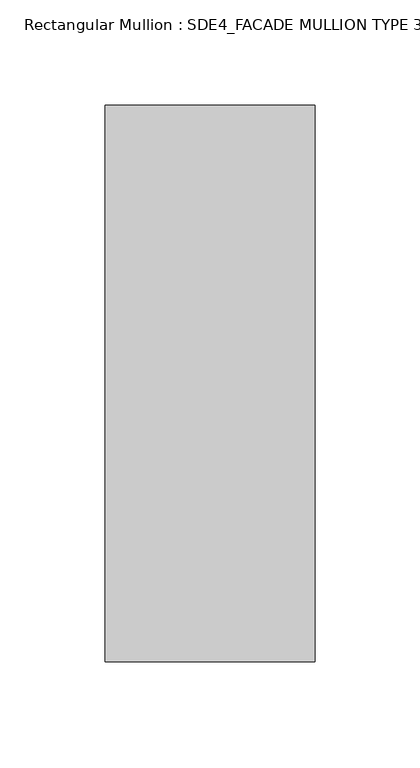
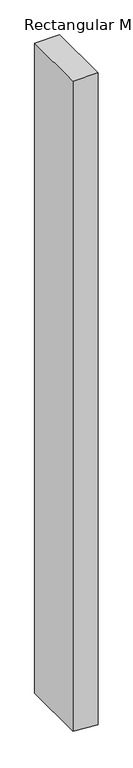
"""IFC4 building model written with IfcOpenShell, lengths in millimetres: member geometry, Rectangular Mullion : SDE4_FACADE MULLION TYPE 3."""

import ifcopenshell
import ifcopenshell.guid

model = None  # the IFC model being written
_history = None  # IfcOwnerHistory: only IFC2X3 demands one
_inside = {}  # id of a spatial element -> (the spatial element, [elements in it])
_under = {}  # id of a project, library or spatial element -> (it, [spatial elements below it])
_declared = {}  # id of a project -> (the project, [libraries it declares])
_typed = {}  # id of a type object -> (the type object, [elements of that type])
_made_of = {}  # id of a material, layer set ... -> (it, [elements and type objects made of it])


def new_model(schema):
    """Start an empty IFC model of exactly this schema.

    Asked for "IFC4X3", IfcOpenShell would pick the latest addendum, in which some entities
    have other attributes; the version numbers below select the first issue.
    IFC2X3 requires an IfcOwnerHistory on every rooted entity: one is made here for all.
    """
    global model, _history
    if schema == "IFC4X3":
        model = ifcopenshell.file(schema_version=(4, 3, 0, 0))
    else:
        model = ifcopenshell.file(schema=schema)
    _inside.clear()
    _under.clear()
    _declared.clear()
    _typed.clear()
    _made_of.clear()
    _history = None
    if model.schema == "IFC2X3":
        org = make("IfcOrganization", Name="unknown")
        user = make(
            "IfcPersonAndOrganization",
            ThePerson=make("IfcPerson", FamilyName="unknown"),
            TheOrganization=org,
        )
        app = make(
            "IfcApplication",
            ApplicationDeveloper=org,
            Version="unknown",
            ApplicationFullName="unknown",
            ApplicationIdentifier="unknown",
        )
        _history = make(
            "IfcOwnerHistory",
            OwningUser=user,
            OwningApplication=app,
            ChangeAction="ADDED",
            CreationDate=0,
        )
    return model


def make(cls, **values):
    """One entity of the class cls with the attributes given. An attribute that is None is left unset."""
    return model.create_entity(
        cls, **{name: value for name, value in values.items() if value is not None}
    )


def rooted(cls, **values):
    """An entity with a GlobalId (a new one), such as an element, a storey or a relation."""
    return make(cls, GlobalId=ifcopenshell.guid.new(), OwnerHistory=_history, **values)


def si_unit(unit_type, name, prefix=None):
    """IfcSIUnit, for example si_unit("LENGTHUNIT", "METRE", prefix="MILLI")."""
    return make("IfcSIUnit", UnitType=unit_type, Prefix=prefix, Name=name)


def assignment(units):
    """IfcUnitAssignment: the units of a project."""
    return None if units is None else make("IfcUnitAssignment", Units=units)


def point(xyz):
    """IfcCartesianPoint."""
    return None if xyz is None else make("IfcCartesianPoint", Coordinates=xyz)


def direction(xyz):
    """IfcDirection."""
    return None if xyz is None else make("IfcDirection", DirectionRatios=xyz)


def frame(location, z_axis=None, x_axis=None):
    """IfcAxis2Placement3D, a coordinate frame: its origin and axes. An axis left out is left unset."""
    return make(
        "IfcAxis2Placement3D",
        Location=point(location),
        Axis=direction(z_axis),
        RefDirection=direction(x_axis),
    )


def origin():
    """The frame at (0, 0, 0) with its axes left unset."""
    return frame((0.0, 0.0, 0.0))


def place(relative_to, where):
    """IfcLocalPlacement: puts the frame where relative to a parent placement (None: the world)."""
    return make(
        "IfcLocalPlacement", PlacementRelTo=relative_to, RelativePlacement=where
    )


def context(
    kind, dimensions, precision=None, world=None, true_north=None, identifier=None
):
    """IfcGeometricRepresentationContext, for example the 3D "Model" context."""
    return make(
        "IfcGeometricRepresentationContext",
        ContextIdentifier=identifier,
        ContextType=kind,
        CoordinateSpaceDimension=dimensions,
        Precision=precision,
        WorldCoordinateSystem=world,
        TrueNorth=true_north,
    )


def project(units=None, contexts=None):
    """IfcProject with its units and contexts."""
    return rooted(
        "IfcProject",
        Name="project",
        RepresentationContexts=contexts,
        UnitsInContext=assignment(units),
    )


def spatial(cls, under=None, at=None, **own):
    """A site, building, storey or space (cls), placed at a placement, below another one or the project."""
    s = rooted(cls, ObjectPlacement=at, **own)
    if under is not None:
        _under.setdefault(under.id(), (under, []))[1].append(s)
    return s


def polyline(points):
    """IfcPolyline through the points."""
    return make("IfcPolyline", Points=[point(p) for p in points])


def outline(outer, holes=None, kind="AREA"):
    """IfcArbitraryClosedProfileDef: a profile drawn as a closed curve; with holes, ...WithVoids."""
    if holes is None:
        return make("IfcArbitraryClosedProfileDef", ProfileType=kind, OuterCurve=outer)
    return make(
        "IfcArbitraryProfileDefWithVoids",
        ProfileType=kind,
        OuterCurve=outer,
        InnerCurves=holes,
    )


def extrude(swept, where, along, depth):
    """IfcExtrudedAreaSolid: the profile swept, set in the frame where, extruded along a direction by depth."""
    return make(
        "IfcExtrudedAreaSolid",
        SweptArea=swept,
        Position=where,
        ExtrudedDirection=direction(along),
        Depth=depth,
    )


def shape(context_of_items, identifier, shape_type, items):
    """IfcShapeRepresentation: the items that make up one representation, for example the "Body"."""
    return make(
        "IfcShapeRepresentation",
        ContextOfItems=context_of_items,
        RepresentationIdentifier=identifier,
        RepresentationType=shape_type,
        Items=items,
    )


def source(mapping_origin, context_of_items, identifier, shape_type, items):
    """IfcRepresentationMap: a shape defined once, which mapped items show again and again."""
    return make(
        "IfcRepresentationMap",
        MappingOrigin=mapping_origin,
        MappedRepresentation=shape(context_of_items, identifier, shape_type, items),
    )


def transform(
    local_origin,
    x_axis=None,
    y_axis=None,
    z_axis=None,
    scale=None,
    scale2=None,
    scale3=None,
    uniform=True,
):
    """IfcCartesianTransformationOperator3D, or its non-uniform kind. x_axis, y_axis, z_axis: its Axis1, 2, 3."""
    if uniform:
        return make(
            "IfcCartesianTransformationOperator3D",
            Axis1=direction(x_axis),
            Axis2=direction(y_axis),
            LocalOrigin=point(local_origin),
            Scale=scale,
            Axis3=direction(z_axis),
        )
    return make(
        "IfcCartesianTransformationOperator3DnonUniform",
        Axis1=direction(x_axis),
        Axis2=direction(y_axis),
        LocalOrigin=point(local_origin),
        Scale=scale,
        Axis3=direction(z_axis),
        Scale2=scale2,
        Scale3=scale3,
    )


def mapped(mapping_source, mapping_target):
    """IfcMappedItem: shows the shape of a source again, moved by a transform."""
    return make(
        "IfcMappedItem", MappingSource=mapping_source, MappingTarget=mapping_target
    )


def made_of(thing, what):
    """Note that an element or type object is made of a material, layer set ...; save() writes the relation."""
    if what is not None:
        _made_of.setdefault(what.id(), (what, []))[1].append(thing)
    return thing


def element(
    cls,
    number,
    at=None,
    inside=None,
    cuts=None,
    type_object=None,
    material=None,
    context=None,
    identifier="Body",
    shape_type=None,
    held_by="IfcProductDefinitionShape",
    body=None,
    shapes=None,
    **own,
):
    """One element of the class cls, such as IfcWall. Its Tag is "e" and its number.

    at: its placement. inside: the storey or other place that contains it. cuts: it is an
    opening in that element (IfcRelVoidsElement). A single representation is given by context,
    identifier, shape_type and body (its items); several are given by shapes. held_by: the class
    of the entity that holds the representations. save() writes the other relations.
    """
    e = rooted(cls, Tag="e%d" % number, ObjectPlacement=at, **own)
    if body is not None:
        shapes = [shape(context, identifier, shape_type, body)]
    if shapes is not None:
        e.Representation = make(held_by, Representations=shapes)
    if inside is not None:
        _inside.setdefault(inside.id(), (inside, []))[1].append(e)
    if cuts is not None:
        rooted(
            "IfcRelVoidsElement", RelatingBuildingElement=cuts, RelatedOpeningElement=e
        )
    if type_object is not None:
        _typed.setdefault(type_object.id(), (type_object, []))[1].append(e)
    return made_of(e, material)


def aggregate(whole, parts):
    """IfcRelAggregates: a whole, such as a stair, and the parts it consists of."""
    return rooted("IfcRelAggregates", RelatingObject=whole, RelatedObjects=parts)


def save(model, path):
    """Write the relations noted so far, then the file.

    IfcRelAggregates (storeys below a building ...), IfcRelContainedInSpatialStructure (elements
    in a storey), IfcRelDefinesByType, IfcRelAssociatesMaterial and IfcRelDeclares: one each for
    every whole, place, type object, material and project.
    """
    for whole, parts in _under.values():
        aggregate(whole, parts)
    for where, things in _inside.values():
        rooted(
            "IfcRelContainedInSpatialStructure",
            RelatedElements=things,
            RelatingStructure=where,
        )
    for kind, things in _typed.values():
        rooted("IfcRelDefinesByType", RelatedObjects=things, RelatingType=kind)
    for what, things in _made_of.values():
        rooted("IfcRelAssociatesMaterial", RelatedObjects=things, RelatingMaterial=what)
    for by, libraries in _declared.values():
        rooted("IfcRelDeclares", RelatingContext=by, RelatedDefinitions=libraries)
    model.write(path)


def rectangular_mullion_sde4_facade_mullion_type_3_023ff285(model_context):
    return source(origin(), model_context, "Body", "SweptSolid", [
        extrude(outline(polyline([(0.0, 50.0), (0.0, -50.0), (-2744.1896646, -50.0), (-2748.2557436, 3.056508), (-2751.8533409, 50.0), (0.0, 50.0)])), frame((0.0, -132.5, 0.0), z_axis=(0.0, 1.0, 0.0), x_axis=(0.0, 0.0, 1.0)), (0.0, 0.0, 1.0), 265.0),
    ])


if __name__ == "__main__":
    model = new_model("IFC4")
    model_context = context("Model", 3, world=origin())
    ifc_project = project(units=[si_unit("LENGTHUNIT", "METRE", prefix="MILLI")], contexts=[model_context])
    site = spatial("IfcSite", under=ifc_project)
    building = spatial("IfcBuilding", under=site)
    placement = place(None, origin())
    rectangular_mullion_sde4_facade_mullion_type_3_shape = rectangular_mullion_sde4_facade_mullion_type_3_023ff285(model_context)
    element("IfcMember", 1, ObjectType="Rectangular Mullion : SDE4_FACADE MULLION TYPE 3", at=placement, inside=building, context=model_context, shape_type="MappedRepresentation", body=[
        mapped(rectangular_mullion_sde4_facade_mullion_type_3_shape, transform((0.0, 0.0, 0.0), x_axis=(1.0, 0.0, 0.0), y_axis=(0.0, 1.0, 0.0), z_axis=(0.0, 0.0, 1.0))),
    ])
    save(model, "model.ifc")

# Revit data of these elements
# Type "Rectangular Mullion : SDE4_FACADE MULLION TYPE 3"
#   built-in parameter 1007322 = 0.869423 (stored number, unit not read)
#   built-in parameter 1007321 = 0.164042 (stored number, unit not read)
#   built-in parameter 1007320 = 0.164042 (stored number, unit not read)
